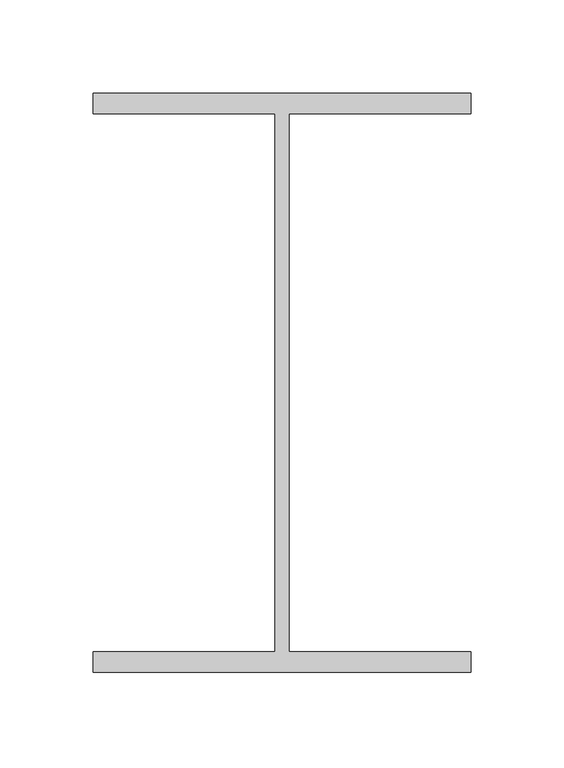
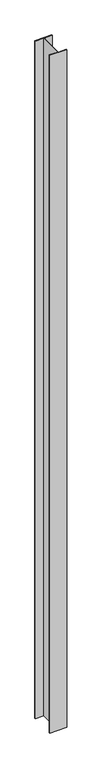
"""IFC4 building model written with IfcOpenShell, lengths in millimetres: proxy geometry, Generic Models 2:Generic Models 2:310765:Generic Models 2:310765 : Generic Models 2:Generic Models 2:310765:77 : Generic Models 2:Generic Models 2:310765:Generic Models 2:310765 : Generic Models 2:Generic Models 2:310765:300385."""

from ifc_helpers import new_model, si_unit, origin, origin_with_axes, place, context, project, spatial, polyline, outline, extrude, source, transform, mapped, element, save


def generic_models_249c6c72(model_context):
    return source(origin(), model_context, "Body", "SweptSolid", [
        extrude(outline(polyline([(579104.5117239, -567621.4913841), (579104.5117239, -567632.5046653), (579006.5828177, -567632.5046653), (579006.5828177, -567921.6281028), (579104.5117239, -567921.6281028), (579104.5117239, -567932.6413841), (578901.2863239, -567932.6413841), (578901.2863239, -567921.6281028), (578999.2406302, -567921.6281028), (578999.2406302, -567632.5046653), (578901.3117239, -567632.5046653), (578901.3117239, -567621.4913841), (579104.5117239, -567621.4913841)])), origin_with_axes(), (0.0, 0.0, 1.0), 8554.7484775),
    ])


if __name__ == "__main__":
    model = new_model("IFC4")
    model_context = context("Model", 3, world=origin())
    ifc_project = project(units=[si_unit("LENGTHUNIT", "METRE", prefix="MILLI")], contexts=[model_context])
    site = spatial("IfcSite", under=ifc_project)
    building = spatial("IfcBuilding", under=site)
    placement = place(None, origin())
    generic_models_shape = generic_models_249c6c72(model_context)
    element("IfcBuildingElementProxy", 1, Name="Generic Models 2:Generic Models 2:310765:Generic Models 2:310765 : Generic Models 2:Generic Models 2:310765:77 : Generic Models 2:Generic Models 2:310765:Generic Models 2:310765 : Generic Models 2:Generic Models 2:310765:300385", ObjectType="Generic Models 2:Generic Models 2:310765:Generic Models 2:310765 : Generic Models 2:Generic Models 2:310765:77 : Generic Models 2:Generic Models 2:310765:Generic Models 2:310765 : Generic Models 2:Generic Models 2:310765:300385", at=placement, inside=building, context=model_context, shape_type="MappedRepresentation", body=[
        mapped(generic_models_shape, transform((0.0, 0.0, 0.0), x_axis=(1.0, 0.0, 0.0), y_axis=(0.0, 1.0, 0.0), z_axis=(0.0, 0.0, 1.0))),
    ])
    save(model, "model.ifc")

# Revit data of these elements
# Type "Generic Models 2:Generic Models 2:310765:Generic Models 2:310765 : Generic Models 2:Generic Models 2:310765:77 : Generic Models 2:Generic Models 2:310765:Generic Models 2:310765 : Generic Models 2:Generic Models 2:310765:300385"
#   NameOverride = "Generic Models 2:Generic Models 2:310765:Generic Models 2:310765 : Generic Models 2:Generic Models 2:310765:300385"
#   ObjectTypeOverride = "Generic Models 2:310765 : Generic Models 2:Generic Models 2:310765"
#   Reference = "Generic Models 2"
#   Tag = "300385"
# Element 1 (IfcBuildingElementProxy, "Generic Models 2:Generic Models 2:310765:Generic Models 2:310765 : Generic Models 2:Generic Models 2:310765:77 : Generic Models 2:Generic Models 2:310765:Generic Models 2:310765 : Generic Models 2:Generic Models 2:310765:300385")
#   Materials on its faces: "STRUCTURAL STEEL - SEE STRUCT. DWGS"
# Materials
#   "STRUCTURAL STEEL - SEE STRUCT. DWGS": class "Metal", colour RGB 189 187 185, transparency 0, Description = "Structural steel 50ksi", Cost = 0
